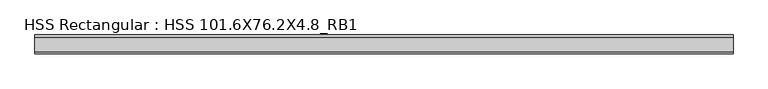
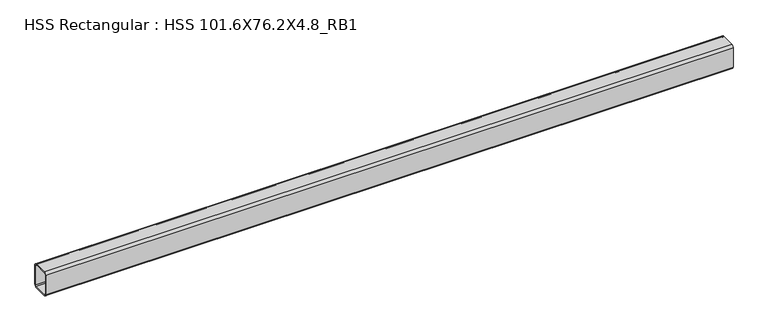
"""IFC4 building model written with IfcOpenShell, lengths in millimetres: beam geometry, HSS Rectangular : HSS 101.6X76.2X4.8_RB1."""

from ifc_helpers import new_model, si_unit, point, frame, frame_2d, origin, place, context, project, spatial, polyline, circle_curve, trimmed, segment, composite_curve, outline, extrude, source, transform, mapped, element, save


def hss_rectangular_hss_101_6x76_2x4_8_rb1_72b12fea(model_context):
    return source(origin(), model_context, "Body", "SweptSolid", [
        extrude(outline(composite_curve([segment(polyline([(38.1, 41.275), (38.1, -41.275)]), True, "CONTINUOUS"), segment(trimmed(circle_curve(frame_2d((28.575, -41.275)), 9.525), [point((38.1, -41.275))], [point((28.575, -50.8))], False, "CARTESIAN"), True, "CONTINUOUS"), segment(polyline([(28.575, -50.8), (-28.575, -50.8)]), True, "CONTINUOUS"), segment(trimmed(circle_curve(frame_2d((-28.575, -41.275)), 9.525), [point((-28.575, -50.8))], [point((-38.1, -41.275))], False, "CARTESIAN"), True, "CONTINUOUS"), segment(polyline([(-38.1, -41.275), (-38.1, 41.275)]), True, "CONTINUOUS"), segment(trimmed(circle_curve(frame_2d((-28.575, 41.275)), 9.525), [point((-38.1, 41.275))], [point((-28.575, 50.8))], False, "CARTESIAN"), True, "CONTINUOUS"), segment(polyline([(-28.575, 50.8), (28.575, 50.8)]), True, "CONTINUOUS"), segment(trimmed(circle_curve(frame_2d((28.575, 41.275)), 9.525), [point((28.575, 50.8))], [point((38.1, 41.275))], False, "CARTESIAN"), True, "CONTINUOUS")], self_intersect=False), holes=[composite_curve([segment(trimmed(circle_curve(frame_2d((-28.575, 41.275)), 4.7625), [point((-28.575, 46.0375))], [point((-33.3375, 41.275))], True, "CARTESIAN"), True, "CONTINUOUS"), segment(polyline([(-33.3375, 41.275), (-33.3375, -41.275)]), True, "CONTINUOUS"), segment(trimmed(circle_curve(frame_2d((-28.575, -41.275)), 4.7625), [point((-33.3375, -41.275))], [point((-28.575, -46.0375))], True, "CARTESIAN"), True, "CONTINUOUS"), segment(polyline([(-28.575, -46.0375), (28.575, -46.0375)]), True, "CONTINUOUS"), segment(trimmed(circle_curve(frame_2d((28.575, -41.275)), 4.7625), [point((28.575, -46.0375))], [point((33.3375, -41.275))], True, "CARTESIAN"), True, "CONTINUOUS"), segment(polyline([(33.3375, -41.275), (33.3375, 41.275)]), True, "CONTINUOUS"), segment(trimmed(circle_curve(frame_2d((28.575, 41.275)), 4.7625), [point((33.3375, 41.275))], [point((28.575, 46.0375))], True, "CARTESIAN"), True, "CONTINUOUS"), segment(polyline([(28.575, 46.0375), (-28.575, 46.0375)]), True, "CONTINUOUS")], self_intersect=False)]), frame((-1410.625, 0.0, 0.0), z_axis=(1.0, 0.0, 0.0), x_axis=(0.0, 1.0, 0.0)), (0.0, 0.0, 1.0), 2795.85),
    ])


if __name__ == "__main__":
    model = new_model("IFC4")
    model_context = context("Model", 3, world=origin())
    ifc_project = project(units=[si_unit("LENGTHUNIT", "METRE", prefix="MILLI")], contexts=[model_context])
    site = spatial("IfcSite", under=ifc_project)
    building = spatial("IfcBuilding", under=site)
    placement = place(None, origin())
    hss_rectangular_hss_101_6x76_2x4_8_rb1_shape = hss_rectangular_hss_101_6x76_2x4_8_rb1_72b12fea(model_context)
    element("IfcBeam", 1, ObjectType="HSS Rectangular : HSS 101.6X76.2X4.8_RB1", at=placement, inside=building, context=model_context, shape_type="MappedRepresentation", body=[
        mapped(hss_rectangular_hss_101_6x76_2x4_8_rb1_shape, transform((0.0, 0.0, 0.0), x_axis=(1.0, 0.0, 0.0), y_axis=(0.0, 1.0, 0.0), z_axis=(0.0, 0.0, 1.0))),
    ])
    save(model, "model.ifc")

# Revit data of these elements
# Type "HSS Rectangular : HSS 101.6X76.2X4.8_RB1"
#   Section Name Key = "HSS 4X3X3/16"
#   Assembly Code = "B10"
#   Width = 7.62 cm
#   Wall Nominal Thickness = 0.4763 cm
#   Wall Design Thickness = 0.442 cm
#   Torsional Moment of Inertia = 260.561 cm⁴
#   Torsional Modulus = 61.2876 cm³
#   Section Area = 14.4516 cm²
#   Plastic Modulus weak axis = 40.3122 cm³
#   Plastic Modulus strong axis = 49.1612 cm³
#   Perimeter = 0.881482 m²/m
#   Outer Fillet = 0.9525 cm
#   Nominal Weight = 12.1285 kgf/m
#   Moment of Inertia weak axis = 131.529 cm⁴
#   Moment of Inertia strong axis = 205.202 cm⁴
#   Inner Fillet = 0.4763 cm
#   Height = 10.16 cm
#   Elastic Modulus weak axis = 34.4128 cm³
#   Elastic Modulus strong axis = 40.476 cm³
#   Centroid Vertical = 5.08 cm
#   Centroid Horizontal = 3.81 cm
#   Length [instance default] = 1524 mm
#   Structural Material [instance default] = Steel ASTM A500, Grade B, Rectangular and Square
#   Principal Axes Angle = 0
# Element 1 (IfcBeam, "HSS Rectangular : HSS 101.6X76.2X4.8_RB1")
#   Structural Material = Steel ASTM A992
#   Materials on its faces: "Steel ASTM A992"
# Materials
#   "Steel ASTM A500, Grade B, Rectangular and Square": class "Metal", colour RGB 199 199 199, transparency 0, Description = "Carbon steel", Cost = 0
#   "Steel ASTM A992": class "Metal", colour RGB 199 199 199, transparency 0, Description = "Structural steel 50ksi", Cost = 0
